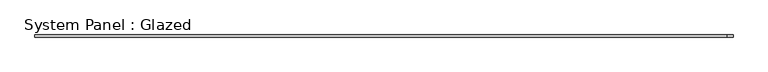
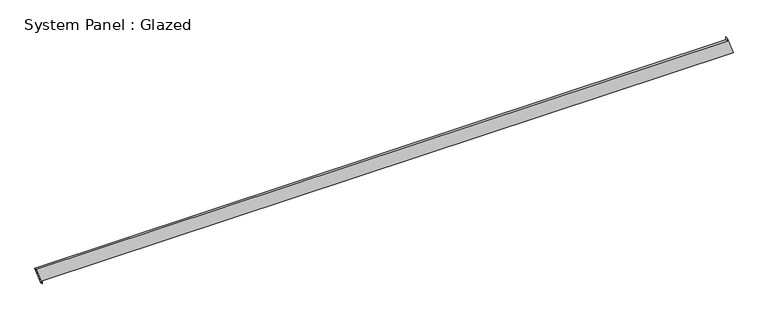
"""IFC4 building model written with IfcOpenShell, lengths in millimetres: plate geometry, System Panel : Glazed."""

from ifc_helpers import new_model, si_unit, frame, origin, place, context, project, spatial, polyline, outline, extrude, source, transform, mapped, element, save


def system_panel_glazed_29c545fd(model_context):
    return source(origin(), model_context, "Body", "SweptSolid", [
        extrude(outline(polyline([(0.0, -3958.6827411), (35.3553391, -3958.6827411), (35.3553391, 4027.7930193), (235.7005018, 3958.9828813), (200.3451627, 3958.98343), (200.2211953, -4027.7930193), (0.0, -3958.6827411)])), frame((0.0, -49.5, 0.0), z_axis=(0.0, 1.0, 0.0), x_axis=(0.0, 0.0, 1.0)), (0.0, 0.0, 1.0), 25.0),
    ])


if __name__ == "__main__":
    model = new_model("IFC4")
    model_context = context("Model", 3, world=origin())
    ifc_project = project(units=[si_unit("LENGTHUNIT", "METRE", prefix="MILLI")], contexts=[model_context])
    site = spatial("IfcSite", under=ifc_project)
    building = spatial("IfcBuilding", under=site)
    placement = place(None, origin())
    system_panel_glazed_shape = system_panel_glazed_29c545fd(model_context)
    element("IfcPlate", 1, ObjectType="System Panel : Glazed", at=placement, inside=building, context=model_context, shape_type="MappedRepresentation", body=[
        mapped(system_panel_glazed_shape, transform((0.0, 0.0, 0.0), x_axis=(1.0, 0.0, 0.0), y_axis=(0.0, 1.0, 0.0), z_axis=(0.0, 0.0, 1.0))),
    ])
    save(model, "model.ifc")

# Revit data of these elements
# Element 1 (IfcPlate, "System Panel : Glazed")
#   Materials on its faces: "Glass"
# Materials
#   "Glass": class "Glass", colour RGB 218 227 224, transparency 0.85, Description = "Soda Lime Glass", Cost = 0
